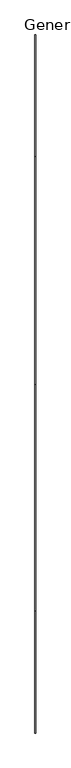
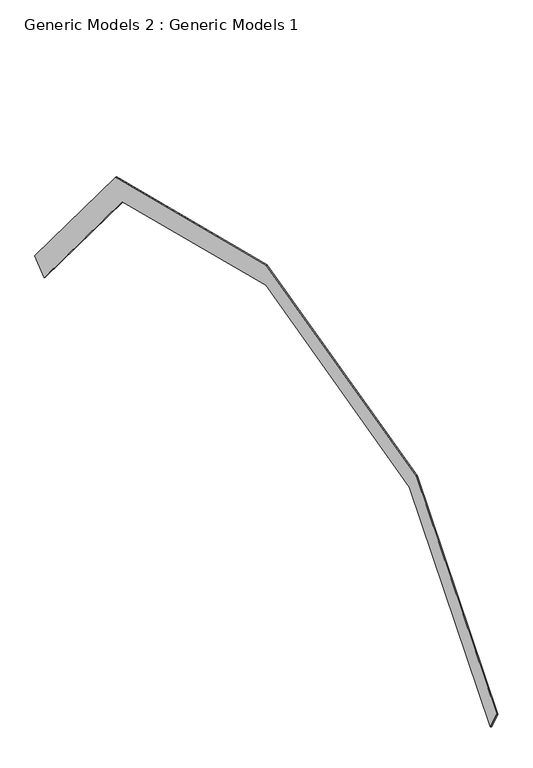
"""IFC4 building model written with IfcOpenShell, lengths in millimetres: proxy geometry, Generic Models 2 : Generic Models 1."""

from ifc_helpers import new_model, si_unit, frame, origin, place, context, project, spatial, polyline, outline, extrude, source, transform, mapped, element, save


def generic_models_2_generic_models_1_059ed1a1(model_context):
    return source(origin(), model_context, "Body", "SweptSolid", [
        extrude(outline(polyline([(11609.9309883, 2984.3405795), (10023.6412719, 4887.8882391), (7113.0570149, 5615.5343034), (4202.4384941, 4887.8796732), (2560.7151338, 2917.8116409), (2434.8673967, 3148.0206952), (4066.3626163, 5105.8149588), (7113.772024, 5867.6673107), (10161.1814316, 5105.8149588), (11797.360301, 3142.4003155), (11609.9309883, 2984.3405795)])), frame((29947.3870052, 0.0, 0.0), z_axis=(1.0, 0.0, 0.0), x_axis=(0.0, 1.0, 0.0)), (0.0, 0.0, 1.0), 13.5023771),
    ])


if __name__ == "__main__":
    model = new_model("IFC4")
    model_context = context("Model", 3, world=origin())
    ifc_project = project(units=[si_unit("LENGTHUNIT", "METRE", prefix="MILLI")], contexts=[model_context])
    site = spatial("IfcSite", under=ifc_project)
    building = spatial("IfcBuilding", under=site)
    placement = place(None, origin())
    generic_models_2_generic_models_1_shape = generic_models_2_generic_models_1_059ed1a1(model_context)
    element("IfcBuildingElementProxy", 1, Name="Generic Models 2 : Generic Models 1", ObjectType="Generic Models 2 : Generic Models 1", at=placement, inside=building, context=model_context, shape_type="MappedRepresentation", body=[
        mapped(generic_models_2_generic_models_1_shape, transform((0.0, 0.0, 0.0), x_axis=(1.0, 0.0, 0.0), y_axis=(0.0, 1.0, 0.0), z_axis=(0.0, 0.0, 1.0))),
    ])
    save(model, "model.ifc")
